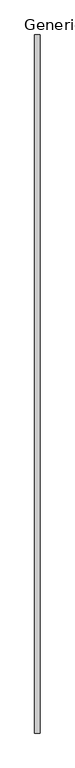
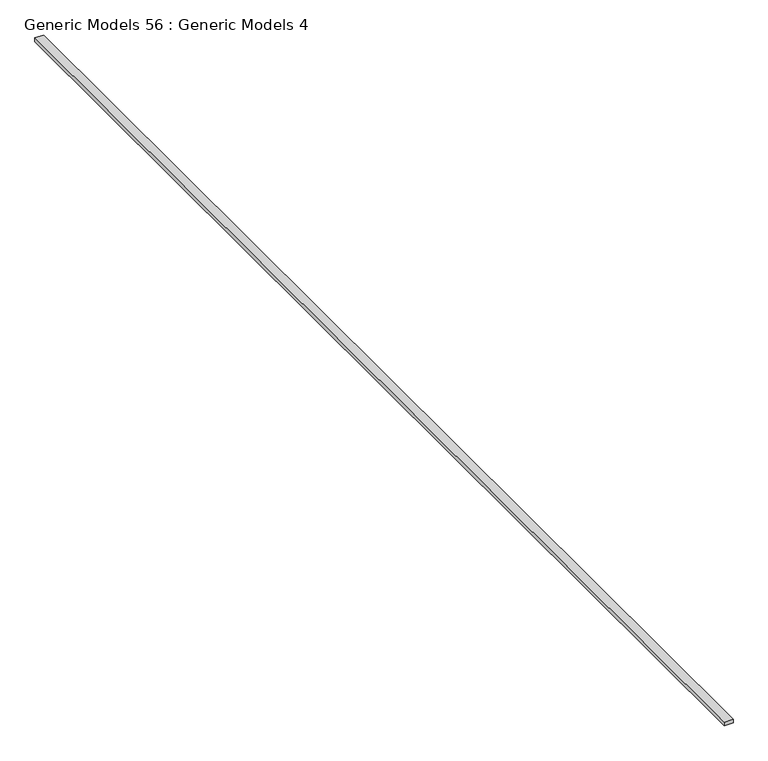
"""IFC4 building model written with IfcOpenShell, lengths in millimetres: proxy geometry, Generic Models 56 : Generic Models 4."""

from ifc_helpers import new_model, si_unit, frame, origin, place, context, project, spatial, polyline, outline, extrude, source, transform, mapped, element, save


def generic_models_56_generic_models_4_a01001ad(model_context):
    return source(origin(), model_context, "Body", "SweptSolid", [
        extrude(outline(polyline([(127040.4410334, 8188.1513704), (127040.4410334, 8327.8513704), (127097.68533, 8327.8513704), (127103.5061634, 8188.1513704), (127040.4410334, 8188.1513704)])), frame((0.0, -6864.9230338, 0.0), z_axis=(0.0, 1.0, 0.0), x_axis=(0.0, 0.0, 1.0)), (0.0, 0.0, 1.0), 18643.6),
    ])


if __name__ == "__main__":
    model = new_model("IFC4")
    model_context = context("Model", 3, world=origin())
    ifc_project = project(units=[si_unit("LENGTHUNIT", "METRE", prefix="MILLI")], contexts=[model_context])
    site = spatial("IfcSite", under=ifc_project)
    building = spatial("IfcBuilding", under=site)
    placement = place(None, origin())
    generic_models_56_generic_models_4_shape = generic_models_56_generic_models_4_a01001ad(model_context)
    element("IfcBuildingElementProxy", 1, Name="Generic Models 56 : Generic Models 4", ObjectType="Generic Models 56 : Generic Models 4", at=placement, inside=building, context=model_context, shape_type="MappedRepresentation", body=[
        mapped(generic_models_56_generic_models_4_shape, transform((0.0, 0.0, 0.0), x_axis=(1.0, 0.0, 0.0), y_axis=(0.0, 1.0, 0.0), z_axis=(0.0, 0.0, 1.0))),
    ])
    save(model, "model.ifc")

# Revit data of these elements
# Element 1 (IfcBuildingElementProxy, "Generic Models 56 : Generic Models 4")
#   Materials on its faces: "_2X BLOCKING AS REQUIRED"
# Materials
#   "_2X BLOCKING AS REQUIRED": class "Generic", colour RGB 177 130 114, transparency 0, Cost = 0
